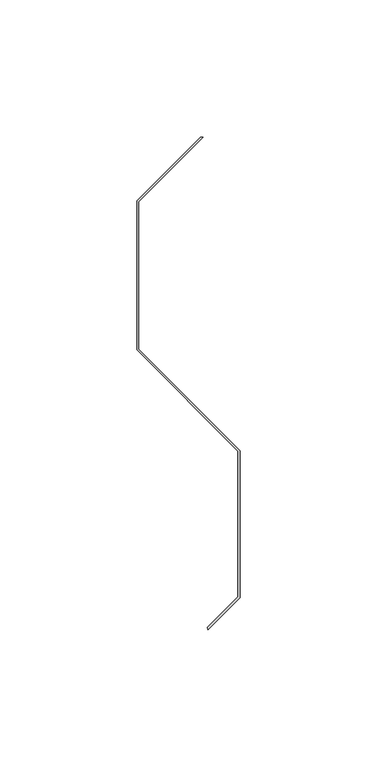
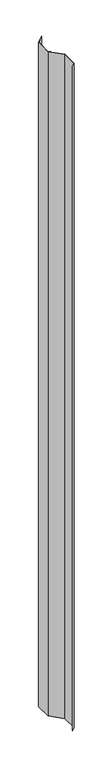
"""IFC4 building model written with IfcOpenShell, lengths in millimetres: proxy geometry, MBCI 7.2-V Panel21 : MBCI 7.2-V Panel-1."""

import ifcopenshell
import ifcopenshell.guid

model = None  # the IFC model being written
_history = None  # IfcOwnerHistory: only IFC2X3 demands one
_inside = {}  # id of a spatial element -> (the spatial element, [elements in it])
_under = {}  # id of a project, library or spatial element -> (it, [spatial elements below it])
_declared = {}  # id of a project -> (the project, [libraries it declares])
_typed = {}  # id of a type object -> (the type object, [elements of that type])
_made_of = {}  # id of a material, layer set ... -> (it, [elements and type objects made of it])


def new_model(schema):
    """Start an empty IFC model of exactly this schema.

    Asked for "IFC4X3", IfcOpenShell would pick the latest addendum, in which some entities
    have other attributes; the version numbers below select the first issue.
    IFC2X3 requires an IfcOwnerHistory on every rooted entity: one is made here for all.
    """
    global model, _history
    if schema == "IFC4X3":
        model = ifcopenshell.file(schema_version=(4, 3, 0, 0))
    else:
        model = ifcopenshell.file(schema=schema)
    _inside.clear()
    _under.clear()
    _declared.clear()
    _typed.clear()
    _made_of.clear()
    _history = None
    if model.schema == "IFC2X3":
        org = make("IfcOrganization", Name="unknown")
        user = make(
            "IfcPersonAndOrganization",
            ThePerson=make("IfcPerson", FamilyName="unknown"),
            TheOrganization=org,
        )
        app = make(
            "IfcApplication",
            ApplicationDeveloper=org,
            Version="unknown",
            ApplicationFullName="unknown",
            ApplicationIdentifier="unknown",
        )
        _history = make(
            "IfcOwnerHistory",
            OwningUser=user,
            OwningApplication=app,
            ChangeAction="ADDED",
            CreationDate=0,
        )
    return model


def make(cls, **values):
    """One entity of the class cls with the attributes given. An attribute that is None is left unset."""
    return model.create_entity(
        cls, **{name: value for name, value in values.items() if value is not None}
    )


def rooted(cls, **values):
    """An entity with a GlobalId (a new one), such as an element, a storey or a relation."""
    return make(cls, GlobalId=ifcopenshell.guid.new(), OwnerHistory=_history, **values)


def si_unit(unit_type, name, prefix=None):
    """IfcSIUnit, for example si_unit("LENGTHUNIT", "METRE", prefix="MILLI")."""
    return make("IfcSIUnit", UnitType=unit_type, Prefix=prefix, Name=name)


def assignment(units):
    """IfcUnitAssignment: the units of a project."""
    return None if units is None else make("IfcUnitAssignment", Units=units)


def point(xyz):
    """IfcCartesianPoint."""
    return None if xyz is None else make("IfcCartesianPoint", Coordinates=xyz)


def direction(xyz):
    """IfcDirection."""
    return None if xyz is None else make("IfcDirection", DirectionRatios=xyz)


def frame(location, z_axis=None, x_axis=None):
    """IfcAxis2Placement3D, a coordinate frame: its origin and axes. An axis left out is left unset."""
    return make(
        "IfcAxis2Placement3D",
        Location=point(location),
        Axis=direction(z_axis),
        RefDirection=direction(x_axis),
    )


def origin():
    """The frame at (0, 0, 0) with its axes left unset."""
    return frame((0.0, 0.0, 0.0))


def place(relative_to, where):
    """IfcLocalPlacement: puts the frame where relative to a parent placement (None: the world)."""
    return make(
        "IfcLocalPlacement", PlacementRelTo=relative_to, RelativePlacement=where
    )


def context(
    kind, dimensions, precision=None, world=None, true_north=None, identifier=None
):
    """IfcGeometricRepresentationContext, for example the 3D "Model" context."""
    return make(
        "IfcGeometricRepresentationContext",
        ContextIdentifier=identifier,
        ContextType=kind,
        CoordinateSpaceDimension=dimensions,
        Precision=precision,
        WorldCoordinateSystem=world,
        TrueNorth=true_north,
    )


def project(units=None, contexts=None):
    """IfcProject with its units and contexts."""
    return rooted(
        "IfcProject",
        Name="project",
        RepresentationContexts=contexts,
        UnitsInContext=assignment(units),
    )


def spatial(cls, under=None, at=None, **own):
    """A site, building, storey or space (cls), placed at a placement, below another one or the project."""
    s = rooted(cls, ObjectPlacement=at, **own)
    if under is not None:
        _under.setdefault(under.id(), (under, []))[1].append(s)
    return s


def polyline(points):
    """IfcPolyline through the points."""
    return make("IfcPolyline", Points=[point(p) for p in points])


def outline(outer, holes=None, kind="AREA"):
    """IfcArbitraryClosedProfileDef: a profile drawn as a closed curve; with holes, ...WithVoids."""
    if holes is None:
        return make("IfcArbitraryClosedProfileDef", ProfileType=kind, OuterCurve=outer)
    return make(
        "IfcArbitraryProfileDefWithVoids",
        ProfileType=kind,
        OuterCurve=outer,
        InnerCurves=holes,
    )


def extrude(swept, where, along, depth):
    """IfcExtrudedAreaSolid: the profile swept, set in the frame where, extruded along a direction by depth."""
    return make(
        "IfcExtrudedAreaSolid",
        SweptArea=swept,
        Position=where,
        ExtrudedDirection=direction(along),
        Depth=depth,
    )


def shape(context_of_items, identifier, shape_type, items):
    """IfcShapeRepresentation: the items that make up one representation, for example the "Body"."""
    return make(
        "IfcShapeRepresentation",
        ContextOfItems=context_of_items,
        RepresentationIdentifier=identifier,
        RepresentationType=shape_type,
        Items=items,
    )


def source(mapping_origin, context_of_items, identifier, shape_type, items):
    """IfcRepresentationMap: a shape defined once, which mapped items show again and again."""
    return make(
        "IfcRepresentationMap",
        MappingOrigin=mapping_origin,
        MappedRepresentation=shape(context_of_items, identifier, shape_type, items),
    )


def transform(
    local_origin,
    x_axis=None,
    y_axis=None,
    z_axis=None,
    scale=None,
    scale2=None,
    scale3=None,
    uniform=True,
):
    """IfcCartesianTransformationOperator3D, or its non-uniform kind. x_axis, y_axis, z_axis: its Axis1, 2, 3."""
    if uniform:
        return make(
            "IfcCartesianTransformationOperator3D",
            Axis1=direction(x_axis),
            Axis2=direction(y_axis),
            LocalOrigin=point(local_origin),
            Scale=scale,
            Axis3=direction(z_axis),
        )
    return make(
        "IfcCartesianTransformationOperator3DnonUniform",
        Axis1=direction(x_axis),
        Axis2=direction(y_axis),
        LocalOrigin=point(local_origin),
        Scale=scale,
        Axis3=direction(z_axis),
        Scale2=scale2,
        Scale3=scale3,
    )


def mapped(mapping_source, mapping_target):
    """IfcMappedItem: shows the shape of a source again, moved by a transform."""
    return make(
        "IfcMappedItem", MappingSource=mapping_source, MappingTarget=mapping_target
    )


def made_of(thing, what):
    """Note that an element or type object is made of a material, layer set ...; save() writes the relation."""
    if what is not None:
        _made_of.setdefault(what.id(), (what, []))[1].append(thing)
    return thing


def element(
    cls,
    number,
    at=None,
    inside=None,
    cuts=None,
    type_object=None,
    material=None,
    context=None,
    identifier="Body",
    shape_type=None,
    held_by="IfcProductDefinitionShape",
    body=None,
    shapes=None,
    **own,
):
    """One element of the class cls, such as IfcWall. Its Tag is "e" and its number.

    at: its placement. inside: the storey or other place that contains it. cuts: it is an
    opening in that element (IfcRelVoidsElement). A single representation is given by context,
    identifier, shape_type and body (its items); several are given by shapes. held_by: the class
    of the entity that holds the representations. save() writes the other relations.
    """
    e = rooted(cls, Tag="e%d" % number, ObjectPlacement=at, **own)
    if body is not None:
        shapes = [shape(context, identifier, shape_type, body)]
    if shapes is not None:
        e.Representation = make(held_by, Representations=shapes)
    if inside is not None:
        _inside.setdefault(inside.id(), (inside, []))[1].append(e)
    if cuts is not None:
        rooted(
            "IfcRelVoidsElement", RelatingBuildingElement=cuts, RelatedOpeningElement=e
        )
    if type_object is not None:
        _typed.setdefault(type_object.id(), (type_object, []))[1].append(e)
    return made_of(e, material)


def aggregate(whole, parts):
    """IfcRelAggregates: a whole, such as a stair, and the parts it consists of."""
    return rooted("IfcRelAggregates", RelatingObject=whole, RelatedObjects=parts)


def save(model, path):
    """Write the relations noted so far, then the file.

    IfcRelAggregates (storeys below a building ...), IfcRelContainedInSpatialStructure (elements
    in a storey), IfcRelDefinesByType, IfcRelAssociatesMaterial and IfcRelDeclares: one each for
    every whole, place, type object, material and project.
    """
    for whole, parts in _under.values():
        aggregate(whole, parts)
    for where, things in _inside.values():
        rooted(
            "IfcRelContainedInSpatialStructure",
            RelatedElements=things,
            RelatingStructure=where,
        )
    for kind, things in _typed.values():
        rooted("IfcRelDefinesByType", RelatedObjects=things, RelatingType=kind)
    for what, things in _made_of.values():
        rooted("IfcRelAssociatesMaterial", RelatedObjects=things, RelatingMaterial=what)
    for by, libraries in _declared.values():
        rooted("IfcRelDeclares", RelatingContext=by, RelatedDefinitions=libraries)
    model.write(path)


def generic_models_c199058d(model_context):
    return source(origin(), model_context, "Body", "SweptSolid", [
        extrude(outline(polyline([(587367.6508364, -533005.919184), (587367.6508364, -533059.500484), (587355.9801137, -533071.1712068), (587355.92509, -533070.3843314), (587367.0555239, -533059.2538975), (587367.0555239, -533006.1657706), (587330.1604364, -532969.2706831), (587330.1604364, -532914.9900192), (587353.3965716, -532891.7538841), (587354.2384706, -532891.7538841), (587330.7557489, -532915.2366057), (587330.7557489, -532969.0240965), (587367.6508364, -533005.919184)])), frame((0.0, 0.0, 51.59375), z_axis=(0.0, 0.0, 1.0), x_axis=(1.0, 0.0, 0.0)), (0.0, 0.0, 1.0), 2386.80625),
    ])


if __name__ == "__main__":
    model = new_model("IFC4")
    model_context = context("Model", 3, world=origin())
    ifc_project = project(units=[si_unit("LENGTHUNIT", "METRE", prefix="MILLI")], contexts=[model_context])
    site = spatial("IfcSite", under=ifc_project)
    building = spatial("IfcBuilding", under=site)
    placement = place(None, origin())
    generic_models_shape = generic_models_c199058d(model_context)
    element("IfcBuildingElementProxy", 1, Name="MBCI 7.2-V Panel21 : MBCI 7.2-V Panel-1", ObjectType="MBCI 7.2-V Panel21 : MBCI 7.2-V Panel-1", at=placement, inside=building, context=model_context, shape_type="MappedRepresentation", body=[
        mapped(generic_models_shape, transform((0.0, 0.0, 0.0), x_axis=(1.0, 0.0, 0.0), y_axis=(0.0, 1.0, 0.0), z_axis=(0.0, 0.0, 1.0))),
    ])
    save(model, "model.ifc")

# Revit data of these elements
# Element 1 (IfcBuildingElementProxy, "MBCI 7.2-V Panel21 : MBCI 7.2-V Panel-1")
#   Materials on its faces: "MTL PANEL"
# Materials
#   "MTL PANEL": class "Generic", colour RGB 239 242 240, transparency 0, Cost = 0
